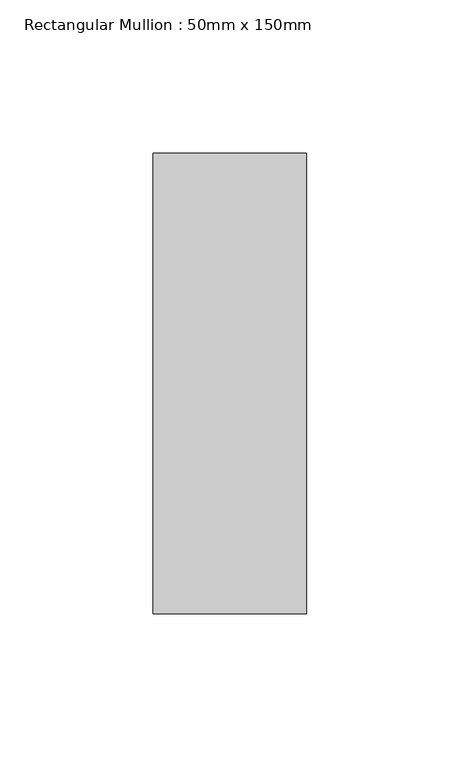
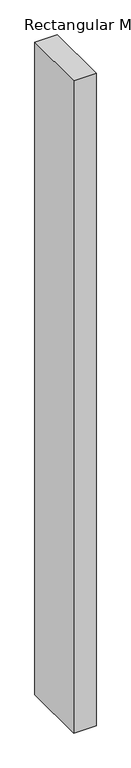
"""IFC4 building model written with IfcOpenShell, lengths in millimetres: member geometry, Rectangular Mullion : 50mm x 150mm."""

from ifc_helpers import new_model, si_unit, frame, origin, place, context, project, spatial, polyline, outline, extrude, source, transform, mapped, element, save


def rectangular_mullion_50mm_x_150mm_bd821fb0(model_context):
    return source(origin(), model_context, "Body", "SweptSolid", [
        extrude(outline(polyline([(0.0, 75.0), (0.0, -75.0), (-50.0, -75.0), (-50.0, 75.0), (0.0, 75.0)])), frame((0.0, 0.0, -1540.0930582), z_axis=(0.0, 0.0, 1.0), x_axis=(1.0, 0.0, 0.0)), (0.0, 0.0, 1.0), 1540.0930582),
    ])


if __name__ == "__main__":
    model = new_model("IFC4")
    model_context = context("Model", 3, world=origin())
    ifc_project = project(units=[si_unit("LENGTHUNIT", "METRE", prefix="MILLI")], contexts=[model_context])
    site = spatial("IfcSite", under=ifc_project)
    building = spatial("IfcBuilding", under=site)
    placement = place(None, origin())
    rectangular_mullion_50mm_x_150mm_shape = rectangular_mullion_50mm_x_150mm_bd821fb0(model_context)
    element("IfcMember", 1, ObjectType="Rectangular Mullion : 50mm x 150mm", at=placement, inside=building, context=model_context, shape_type="MappedRepresentation", body=[
        mapped(rectangular_mullion_50mm_x_150mm_shape, transform((0.0, 0.0, 0.0), x_axis=(1.0, 0.0, 0.0), y_axis=(0.0, 1.0, 0.0), z_axis=(0.0, 0.0, 1.0))),
    ])
    save(model, "model.ifc")

# Revit data of these elements
# Type "Rectangular Mullion : 50mm x 150mm"
#   built-in parameter 1007304 = 0.492126 (stored number, unit not read)
#   built-in parameter 1007301 = 0.082021 (stored number, unit not read)
#   built-in parameter 1007300 = 0.082021 (stored number, unit not read)
# Element 1 (IfcMember, "Rectangular Mullion : 50mm x 150mm")
#   Materials on its faces: "Aluminum"
# Materials
#   "Aluminum": class "Metal", colour RGB 244 244 244, transparency 0, Description = "Aluminum 6061", Cost = 0
